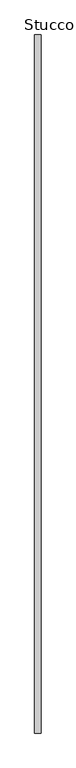
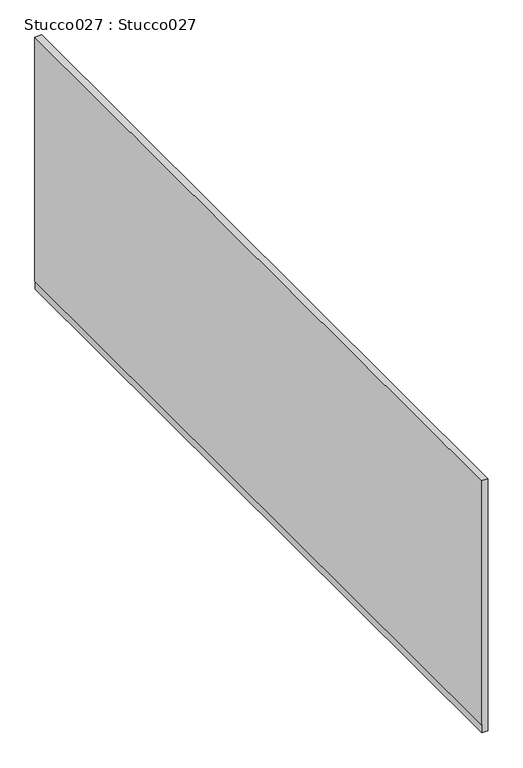
"""IFC4 building model written with IfcOpenShell, lengths in millimetres: proxy geometry, Stucco027 : Stucco027."""

from ifc_helpers import new_model, si_unit, frame, origin, place, context, project, spatial, polyline, outline, extrude, source, transform, mapped, element, save


def stucco027_stucco027_9883634e(model_context):
    return source(origin(), model_context, "Body", "SweptSolid", [
        extrude(outline(polyline([(39567.688258, -5021.258828), (39567.688258, -5019.9730663), (39545.1576447, -5019.9730663), (39545.1576447, -5003.4786233), (40234.4061757, -5003.4786233), (40234.4061757, -5021.258828), (39567.688258, -5021.258828)])), frame((0.0, -1052.8905835, 0.0), z_axis=(0.0, 1.0, 0.0), x_axis=(0.0, 0.0, 1.0)), (0.0, 0.0, 1.0), 2000.0),
    ])


if __name__ == "__main__":
    model = new_model("IFC4")
    model_context = context("Model", 3, world=origin())
    ifc_project = project(units=[si_unit("LENGTHUNIT", "METRE", prefix="MILLI")], contexts=[model_context])
    site = spatial("IfcSite", under=ifc_project)
    building = spatial("IfcBuilding", under=site)
    placement = place(None, origin())
    stucco027_stucco027_shape = stucco027_stucco027_9883634e(model_context)
    element("IfcBuildingElementProxy", 1, Name="Stucco027 : Stucco027", ObjectType="Stucco027 : Stucco027", at=placement, inside=building, context=model_context, shape_type="MappedRepresentation", body=[
        mapped(stucco027_stucco027_shape, transform((0.0, 0.0, 0.0), x_axis=(1.0, 0.0, 0.0), y_axis=(0.0, 1.0, 0.0), z_axis=(0.0, 0.0, 1.0))),
    ])
    save(model, "model.ifc")

# Revit data of these elements
# Type "Stucco027 : Stucco027"
#   NameOverride = "Stucco027"
# Element 1 (IfcBuildingElementProxy, "Stucco027 : Stucco027")
#   Materials on its faces: "7/8\" SMOOTH TROWEL EXTERIOR STUCCO"
# Materials
#   "7/8\" SMOOTH TROWEL EXTERIOR STUCCO": class "Unassigned", colour RGB 255 255 255, transparency 0, Cost = 0
